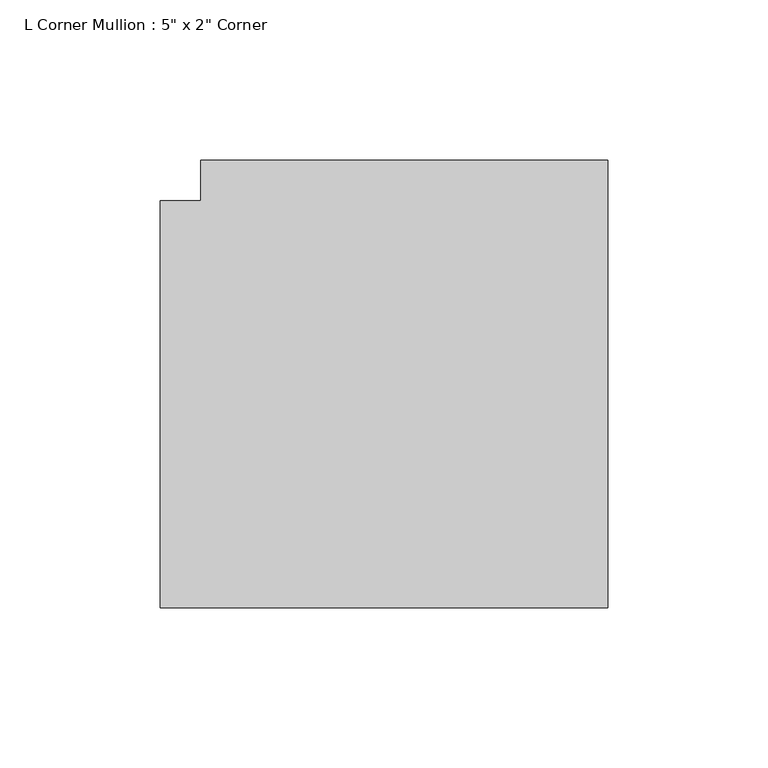
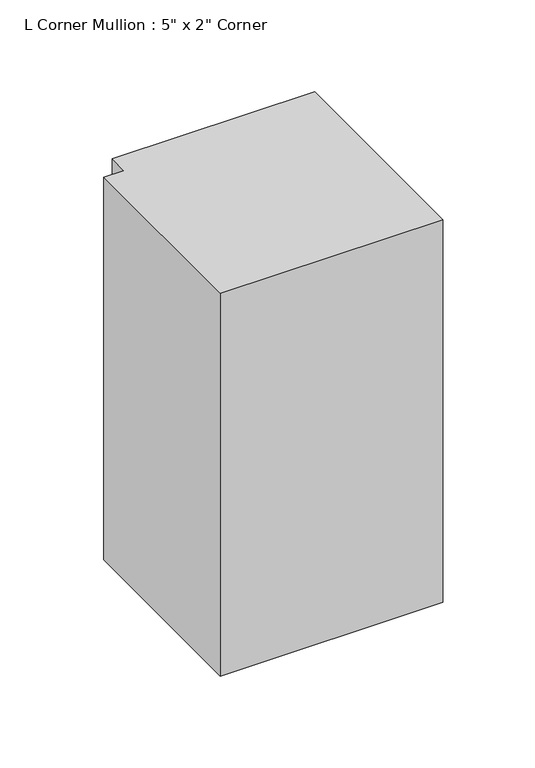
"""IFC4 building model written with IfcOpenShell, lengths in millimetres: member geometry."""

from ifc_helpers import new_model, si_unit, frame, origin, place, context, project, spatial, polyline, outline, extrude, source, transform, mapped, element, save


def member_efed6cf7(model_context):
    return source(origin(), model_context, "Body", "SweptSolid", [
        extrude(outline(polyline([(63.5, 76.2), (63.5, -63.5), (-76.2, -63.5), (-76.2, 63.5), (-63.5, 63.5), (-63.5, 76.2), (63.5, 76.2)])), frame((0.0, 0.0, -254.0), z_axis=(0.0, 0.0, 1.0), x_axis=(1.0, 0.0, 0.0)), (0.0, 0.0, 1.0), 254.0),
    ])


if __name__ == "__main__":
    model = new_model("IFC4")
    model_context = context("Model", 3, world=origin())
    ifc_project = project(units=[si_unit("LENGTHUNIT", "METRE", prefix="MILLI")], contexts=[model_context])
    site = spatial("IfcSite", under=ifc_project)
    building = spatial("IfcBuilding", under=site)
    placement = place(None, origin())
    member_shape = member_efed6cf7(model_context)
    element("IfcMember", 1, ObjectType="L Corner Mullion : 5\" x 2\" Corner", at=placement, inside=building, context=model_context, shape_type="MappedRepresentation", body=[
        mapped(member_shape, transform((0.0, 0.0, 0.0), x_axis=(1.0, 0.0, 0.0), y_axis=(0.0, 1.0, 0.0), z_axis=(0.0, 0.0, 1.0))),
    ])
    save(model, "model.ifc")

# Revit data of these elements
# Type "L Corner Mullion : 5\" x 2\" Corner"
#   built-in parameter 1007355 = 0.25 (stored number, unit not read)
#   built-in parameter 1007354 = 0.25 (stored number, unit not read)
#   built-in parameter 1007304 = 0.416667 (stored number, unit not read)
# Element 1 (IfcMember, "L Corner Mullion : 5\" x 2\" Corner")
#   Materials on its faces: "Metal - Aluminum"
# Materials
#   "Metal - Aluminum": class "Metal", colour RGB 109 108 108, transparency 0
